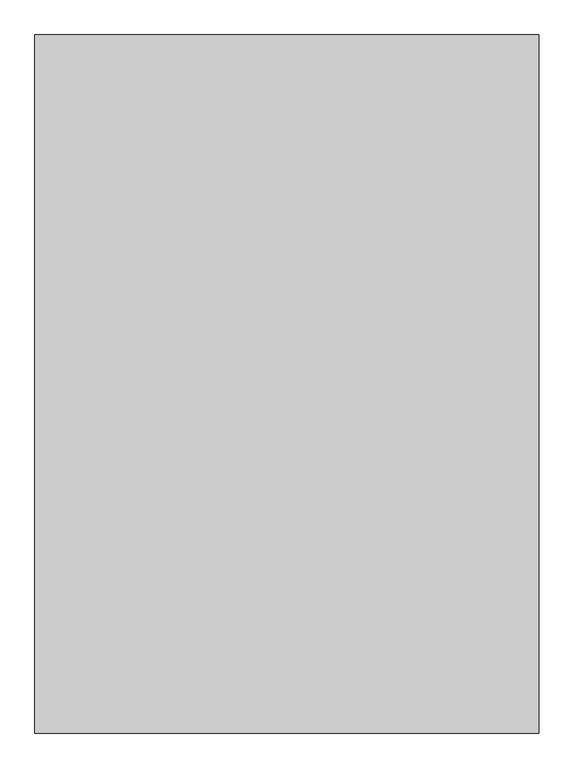
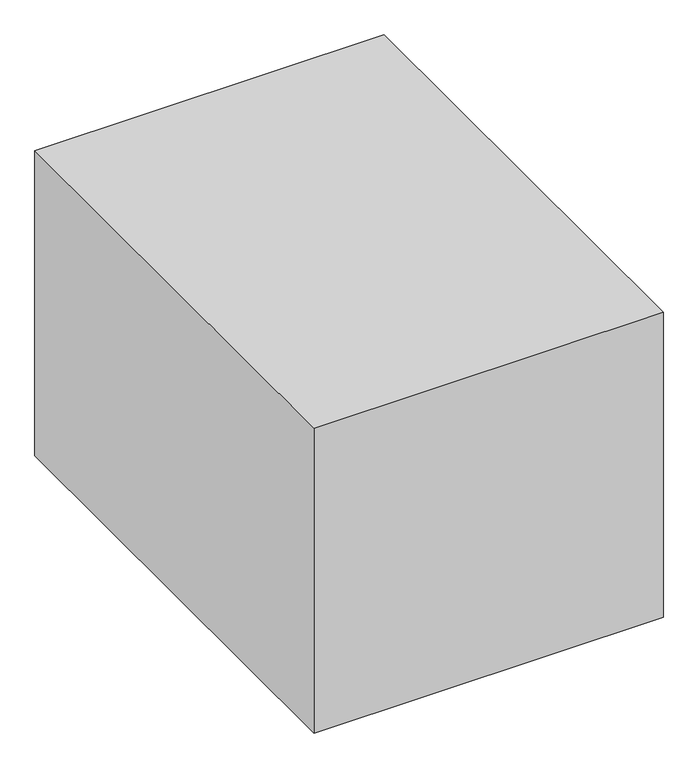
"""IFC4 building model written with IfcOpenShell, lengths in millimetres: proxy geometry, Space Planning Box_hec : Space Planning Box_hec."""

import ifcopenshell
import ifcopenshell.guid

model = None  # the IFC model being written
_history = None  # IfcOwnerHistory: only IFC2X3 demands one
_inside = {}  # id of a spatial element -> (the spatial element, [elements in it])
_under = {}  # id of a project, library or spatial element -> (it, [spatial elements below it])
_declared = {}  # id of a project -> (the project, [libraries it declares])
_typed = {}  # id of a type object -> (the type object, [elements of that type])
_made_of = {}  # id of a material, layer set ... -> (it, [elements and type objects made of it])


def new_model(schema):
    """Start an empty IFC model of exactly this schema.

    Asked for "IFC4X3", IfcOpenShell would pick the latest addendum, in which some entities
    have other attributes; the version numbers below select the first issue.
    IFC2X3 requires an IfcOwnerHistory on every rooted entity: one is made here for all.
    """
    global model, _history
    if schema == "IFC4X3":
        model = ifcopenshell.file(schema_version=(4, 3, 0, 0))
    else:
        model = ifcopenshell.file(schema=schema)
    _inside.clear()
    _under.clear()
    _declared.clear()
    _typed.clear()
    _made_of.clear()
    _history = None
    if model.schema == "IFC2X3":
        org = make("IfcOrganization", Name="unknown")
        user = make(
            "IfcPersonAndOrganization",
            ThePerson=make("IfcPerson", FamilyName="unknown"),
            TheOrganization=org,
        )
        app = make(
            "IfcApplication",
            ApplicationDeveloper=org,
            Version="unknown",
            ApplicationFullName="unknown",
            ApplicationIdentifier="unknown",
        )
        _history = make(
            "IfcOwnerHistory",
            OwningUser=user,
            OwningApplication=app,
            ChangeAction="ADDED",
            CreationDate=0,
        )
    return model


def make(cls, **values):
    """One entity of the class cls with the attributes given. An attribute that is None is left unset."""
    return model.create_entity(
        cls, **{name: value for name, value in values.items() if value is not None}
    )


def rooted(cls, **values):
    """An entity with a GlobalId (a new one), such as an element, a storey or a relation."""
    return make(cls, GlobalId=ifcopenshell.guid.new(), OwnerHistory=_history, **values)


def si_unit(unit_type, name, prefix=None):
    """IfcSIUnit, for example si_unit("LENGTHUNIT", "METRE", prefix="MILLI")."""
    return make("IfcSIUnit", UnitType=unit_type, Prefix=prefix, Name=name)


def assignment(units):
    """IfcUnitAssignment: the units of a project."""
    return None if units is None else make("IfcUnitAssignment", Units=units)


def point(xyz):
    """IfcCartesianPoint."""
    return None if xyz is None else make("IfcCartesianPoint", Coordinates=xyz)


def direction(xyz):
    """IfcDirection."""
    return None if xyz is None else make("IfcDirection", DirectionRatios=xyz)


def frame(location, z_axis=None, x_axis=None):
    """IfcAxis2Placement3D, a coordinate frame: its origin and axes. An axis left out is left unset."""
    return make(
        "IfcAxis2Placement3D",
        Location=point(location),
        Axis=direction(z_axis),
        RefDirection=direction(x_axis),
    )


def origin():
    """The frame at (0, 0, 0) with its axes left unset."""
    return frame((0.0, 0.0, 0.0))


def origin_with_axes():
    """The frame at (0, 0, 0) with the z axis (0, 0, 1) and the x axis (1, 0, 0) written out."""
    return frame((0.0, 0.0, 0.0), z_axis=(0.0, 0.0, 1.0), x_axis=(1.0, 0.0, 0.0))


def place(relative_to, where):
    """IfcLocalPlacement: puts the frame where relative to a parent placement (None: the world)."""
    return make(
        "IfcLocalPlacement", PlacementRelTo=relative_to, RelativePlacement=where
    )


def context(
    kind, dimensions, precision=None, world=None, true_north=None, identifier=None
):
    """IfcGeometricRepresentationContext, for example the 3D "Model" context."""
    return make(
        "IfcGeometricRepresentationContext",
        ContextIdentifier=identifier,
        ContextType=kind,
        CoordinateSpaceDimension=dimensions,
        Precision=precision,
        WorldCoordinateSystem=world,
        TrueNorth=true_north,
    )


def project(units=None, contexts=None):
    """IfcProject with its units and contexts."""
    return rooted(
        "IfcProject",
        Name="project",
        RepresentationContexts=contexts,
        UnitsInContext=assignment(units),
    )


def spatial(cls, under=None, at=None, **own):
    """A site, building, storey or space (cls), placed at a placement, below another one or the project."""
    s = rooted(cls, ObjectPlacement=at, **own)
    if under is not None:
        _under.setdefault(under.id(), (under, []))[1].append(s)
    return s


def polyline(points):
    """IfcPolyline through the points."""
    return make("IfcPolyline", Points=[point(p) for p in points])


def outline(outer, holes=None, kind="AREA"):
    """IfcArbitraryClosedProfileDef: a profile drawn as a closed curve; with holes, ...WithVoids."""
    if holes is None:
        return make("IfcArbitraryClosedProfileDef", ProfileType=kind, OuterCurve=outer)
    return make(
        "IfcArbitraryProfileDefWithVoids",
        ProfileType=kind,
        OuterCurve=outer,
        InnerCurves=holes,
    )


def extrude(swept, where, along, depth):
    """IfcExtrudedAreaSolid: the profile swept, set in the frame where, extruded along a direction by depth."""
    return make(
        "IfcExtrudedAreaSolid",
        SweptArea=swept,
        Position=where,
        ExtrudedDirection=direction(along),
        Depth=depth,
    )


def shape(context_of_items, identifier, shape_type, items):
    """IfcShapeRepresentation: the items that make up one representation, for example the "Body"."""
    return make(
        "IfcShapeRepresentation",
        ContextOfItems=context_of_items,
        RepresentationIdentifier=identifier,
        RepresentationType=shape_type,
        Items=items,
    )


def source(mapping_origin, context_of_items, identifier, shape_type, items):
    """IfcRepresentationMap: a shape defined once, which mapped items show again and again."""
    return make(
        "IfcRepresentationMap",
        MappingOrigin=mapping_origin,
        MappedRepresentation=shape(context_of_items, identifier, shape_type, items),
    )


def transform(
    local_origin,
    x_axis=None,
    y_axis=None,
    z_axis=None,
    scale=None,
    scale2=None,
    scale3=None,
    uniform=True,
):
    """IfcCartesianTransformationOperator3D, or its non-uniform kind. x_axis, y_axis, z_axis: its Axis1, 2, 3."""
    if uniform:
        return make(
            "IfcCartesianTransformationOperator3D",
            Axis1=direction(x_axis),
            Axis2=direction(y_axis),
            LocalOrigin=point(local_origin),
            Scale=scale,
            Axis3=direction(z_axis),
        )
    return make(
        "IfcCartesianTransformationOperator3DnonUniform",
        Axis1=direction(x_axis),
        Axis2=direction(y_axis),
        LocalOrigin=point(local_origin),
        Scale=scale,
        Axis3=direction(z_axis),
        Scale2=scale2,
        Scale3=scale3,
    )


def mapped(mapping_source, mapping_target):
    """IfcMappedItem: shows the shape of a source again, moved by a transform."""
    return make(
        "IfcMappedItem", MappingSource=mapping_source, MappingTarget=mapping_target
    )


def made_of(thing, what):
    """Note that an element or type object is made of a material, layer set ...; save() writes the relation."""
    if what is not None:
        _made_of.setdefault(what.id(), (what, []))[1].append(thing)
    return thing


def element(
    cls,
    number,
    at=None,
    inside=None,
    cuts=None,
    type_object=None,
    material=None,
    context=None,
    identifier="Body",
    shape_type=None,
    held_by="IfcProductDefinitionShape",
    body=None,
    shapes=None,
    **own,
):
    """One element of the class cls, such as IfcWall. Its Tag is "e" and its number.

    at: its placement. inside: the storey or other place that contains it. cuts: it is an
    opening in that element (IfcRelVoidsElement). A single representation is given by context,
    identifier, shape_type and body (its items); several are given by shapes. held_by: the class
    of the entity that holds the representations. save() writes the other relations.
    """
    e = rooted(cls, Tag="e%d" % number, ObjectPlacement=at, **own)
    if body is not None:
        shapes = [shape(context, identifier, shape_type, body)]
    if shapes is not None:
        e.Representation = make(held_by, Representations=shapes)
    if inside is not None:
        _inside.setdefault(inside.id(), (inside, []))[1].append(e)
    if cuts is not None:
        rooted(
            "IfcRelVoidsElement", RelatingBuildingElement=cuts, RelatedOpeningElement=e
        )
    if type_object is not None:
        _typed.setdefault(type_object.id(), (type_object, []))[1].append(e)
    return made_of(e, material)


def aggregate(whole, parts):
    """IfcRelAggregates: a whole, such as a stair, and the parts it consists of."""
    return rooted("IfcRelAggregates", RelatingObject=whole, RelatedObjects=parts)


def save(model, path):
    """Write the relations noted so far, then the file.

    IfcRelAggregates (storeys below a building ...), IfcRelContainedInSpatialStructure (elements
    in a storey), IfcRelDefinesByType, IfcRelAssociatesMaterial and IfcRelDeclares: one each for
    every whole, place, type object, material and project.
    """
    for whole, parts in _under.values():
        aggregate(whole, parts)
    for where, things in _inside.values():
        rooted(
            "IfcRelContainedInSpatialStructure",
            RelatedElements=things,
            RelatingStructure=where,
        )
    for kind, things in _typed.values():
        rooted("IfcRelDefinesByType", RelatedObjects=things, RelatingType=kind)
    for what, things in _made_of.values():
        rooted("IfcRelAssociatesMaterial", RelatedObjects=things, RelatingMaterial=what)
    for by, libraries in _declared.values():
        rooted("IfcRelDeclares", RelatingContext=by, RelatedDefinitions=libraries)
    model.write(path)


def generic_models_1d705098(model_context):
    return source(origin(), model_context, "Body", "SweptSolid", [
        extrude(outline(polyline([(3250.0, 4500.0), (3250.0, -4500.0), (-3250.0, -4500.0), (-3250.0, 4500.0), (3250.0, 4500.0)])), origin_with_axes(), (0.0, 0.0, 1.0), 6000.0),
    ])


if __name__ == "__main__":
    model = new_model("IFC4")
    model_context = context("Model", 3, world=origin())
    ifc_project = project(units=[si_unit("LENGTHUNIT", "METRE", prefix="MILLI")], contexts=[model_context])
    site = spatial("IfcSite", under=ifc_project)
    building = spatial("IfcBuilding", under=site)
    placement = place(None, origin())
    generic_models_shape = generic_models_1d705098(model_context)
    element("IfcBuildingElementProxy", 1, Name="Space Planning Box_hec : Space Planning Box_hec", ObjectType="Space Planning Box_hec : Space Planning Box_hec", at=placement, inside=building, context=model_context, shape_type="MappedRepresentation", body=[
        mapped(generic_models_shape, transform((0.0, 0.0, 0.0), x_axis=(1.0, 0.0, 0.0), y_axis=(0.0, 1.0, 0.0), z_axis=(0.0, 0.0, 1.0))),
    ])
    save(model, "model.ifc")

# Revit data of these elements
# Type "Space Planning Box_hec : Space Planning Box_hec"
#   Type Comments = "..."
#   Room Name [instance default] = "?"
#   Interior Finish [instance default] = ""
#   Exterior Finish [instance default] = ""
#   Department [instance default] = ""
#   Assembly Code = "..."
#   Width [instance default] = 1524 mm
#   Program Area [instance default] = 0.00 m²
#   Length [instance default] = 1524 mm
#   Height [instance default] = 1524 mm
#   Area [instance default] = 2.32258 m²
#   Fill Color [instance default] = Cyan
#   Default Elevation = 0
# Element 1 (IfcBuildingElementProxy, "Space Planning Box_hec : Space Planning Box_hec")
#   Room Name = "Switchgear Room"
#   Interior Finish = "IF1"
#   Exterior Finish = "EF1"
#   Department = "EL"
#   Width = 6500 mm
#   Program Area = 58.50 m²
#   Length = 9000 mm
#   Height = 6000 mm
#   Area = 58.50 m²
#   Fill Color = Blue
#   Materials on its faces: "Blue"
# Materials
#   "Cyan": class "Generic", colour RGB 0 255 255, transparency 0.2, Cost = 0
#   "Blue": class "Generic", colour RGB 0 0 255, transparency 0.2, Cost = 0
